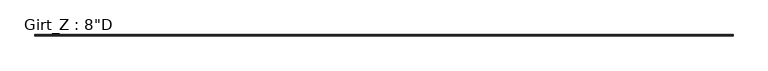
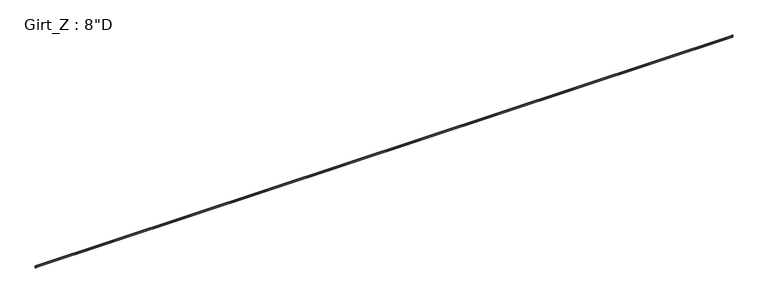
"""IFC4 building model written with IfcOpenShell, lengths in millimetres: beam geometry."""

from ifc_helpers import new_model, si_unit, point, frame, frame_2d, origin, place, context, project, spatial, polyline, circle_curve, trimmed, segment, composite_curve, outline, extrude, source, transform, mapped, element, save


def beam_1eed4de9(model_context):
    return source(origin(), model_context, "Body", "SweptSolid", [
        extrude(outline(composite_curve([segment(polyline([(-63.5, 101.6), (-3.3734375, 101.6)]), True, "CONTINUOUS"), segment(trimmed(circle_curve(frame_2d((-3.3734375, 96.8375)), 4.7625), [point((-3.3734375, 101.6))], [point((1.3890625, 96.8375))], False, "CARTESIAN"), True, "CONTINUOUS"), segment(polyline([(1.3890625, 96.8375), (1.3890625, -96.8389339)]), True, "CONTINUOUS"), segment(trimmed(circle_curve(frame_2d((3.3748024, -96.8389339)), 1.9857399), [point((1.3890625, -96.8389339))], [point((3.2694106, -98.821875))], True, "CARTESIAN"), True, "CONTINUOUS"), segment(polyline([(3.2694106, -98.821875), (62.204539, -98.821875), (73.6169367, -85.221109), (75.745104, -87.0068534), (63.5, -101.6), (3.3734375, -101.6)]), True, "CONTINUOUS"), segment(trimmed(circle_curve(frame_2d((3.3734375, -96.8375)), 4.7625), [point((3.3734375, -101.6))], [point((-1.3890625, -96.8375))], False, "CARTESIAN"), True, "CONTINUOUS"), segment(polyline([(-1.3890625, -96.8375), (-1.3890625, 96.8381931)]), True, "CONTINUOUS"), segment(trimmed(circle_curve(frame_2d((-3.3741066, 96.8381931)), 1.9850441), [point((-1.3890625, 96.8381931))], [point((-3.3005807, 98.821875))], True, "CARTESIAN"), True, "CONTINUOUS"), segment(polyline([(-3.3005807, 98.821875), (-62.204539, 98.821875), (-73.6169367, 85.221109), (-75.745104, 87.0068534), (-63.5, 101.6)]), True, "CONTINUOUS")], self_intersect=False)), frame((-36879.0884766, 0.0, 0.0), z_axis=(1.0, 0.0, 0.0), x_axis=(0.0, 1.0, 0.0)), (0.0, 0.0, 1.0), 73758.1769531),
    ])


if __name__ == "__main__":
    model = new_model("IFC4")
    model_context = context("Model", 3, world=origin())
    ifc_project = project(units=[si_unit("LENGTHUNIT", "METRE", prefix="MILLI")], contexts=[model_context])
    site = spatial("IfcSite", under=ifc_project)
    building = spatial("IfcBuilding", under=site)
    placement = place(None, origin())
    beam_shape = beam_1eed4de9(model_context)
    element("IfcBeam", 1, ObjectType="Girt_Z : 8\"D", at=placement, inside=building, context=model_context, shape_type="MappedRepresentation", body=[
        mapped(beam_shape, transform((0.0, 0.0, 0.0), x_axis=(1.0, 0.0, 0.0), y_axis=(0.0, 1.0, 0.0), z_axis=(0.0, 0.0, 1.0))),
    ])
    save(model, "model.ifc")

# Revit data of these elements
# Type "Girt_Z : 8\"D"
#   Web_Thickness = 0' - 0 7/64"
#   Length [instance default] = 10' - 0"
#   Leg_1 = 0' - 2 1/2"
#   Height = 0' - 8"
#   Structural Material [instance default] = none
# Element 1 (IfcBeam, "Girt_Z : 8\"D")
#   Structural Material = Steel
#   Materials on its faces: "Steel"
# Materials
#   "Steel": class "Metal", colour RGB 118 118 114, transparency 0, Description = "Steel, mill finish", Cost = 0
